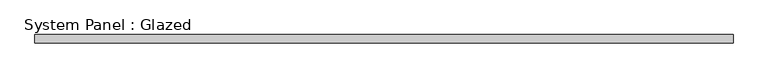
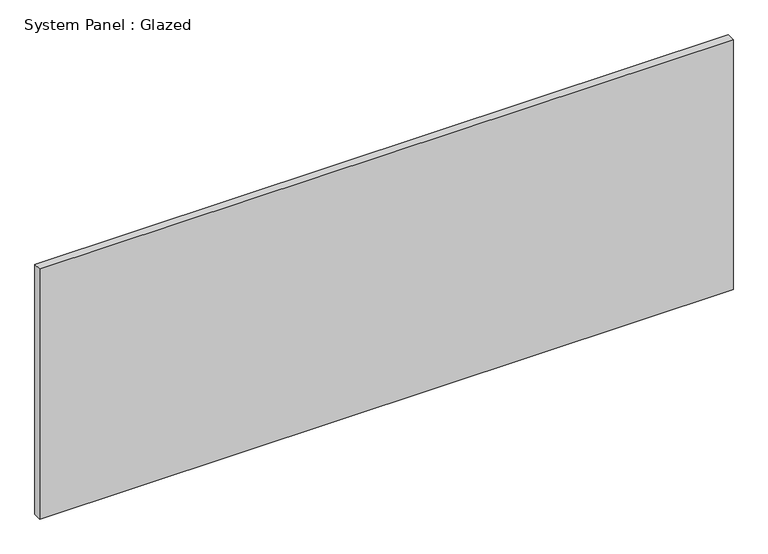
"""IFC4 building model written with IfcOpenShell, lengths in millimetres: plate geometry, System Panel : Glazed."""

import ifcopenshell
import ifcopenshell.guid

model = None  # the IFC model being written
_history = None  # IfcOwnerHistory: only IFC2X3 demands one
_inside = {}  # id of a spatial element -> (the spatial element, [elements in it])
_under = {}  # id of a project, library or spatial element -> (it, [spatial elements below it])
_declared = {}  # id of a project -> (the project, [libraries it declares])
_typed = {}  # id of a type object -> (the type object, [elements of that type])
_made_of = {}  # id of a material, layer set ... -> (it, [elements and type objects made of it])


def new_model(schema):
    """Start an empty IFC model of exactly this schema.

    Asked for "IFC4X3", IfcOpenShell would pick the latest addendum, in which some entities
    have other attributes; the version numbers below select the first issue.
    IFC2X3 requires an IfcOwnerHistory on every rooted entity: one is made here for all.
    """
    global model, _history
    if schema == "IFC4X3":
        model = ifcopenshell.file(schema_version=(4, 3, 0, 0))
    else:
        model = ifcopenshell.file(schema=schema)
    _inside.clear()
    _under.clear()
    _declared.clear()
    _typed.clear()
    _made_of.clear()
    _history = None
    if model.schema == "IFC2X3":
        org = make("IfcOrganization", Name="unknown")
        user = make(
            "IfcPersonAndOrganization",
            ThePerson=make("IfcPerson", FamilyName="unknown"),
            TheOrganization=org,
        )
        app = make(
            "IfcApplication",
            ApplicationDeveloper=org,
            Version="unknown",
            ApplicationFullName="unknown",
            ApplicationIdentifier="unknown",
        )
        _history = make(
            "IfcOwnerHistory",
            OwningUser=user,
            OwningApplication=app,
            ChangeAction="ADDED",
            CreationDate=0,
        )
    return model


def make(cls, **values):
    """One entity of the class cls with the attributes given. An attribute that is None is left unset."""
    return model.create_entity(
        cls, **{name: value for name, value in values.items() if value is not None}
    )


def rooted(cls, **values):
    """An entity with a GlobalId (a new one), such as an element, a storey or a relation."""
    return make(cls, GlobalId=ifcopenshell.guid.new(), OwnerHistory=_history, **values)


def si_unit(unit_type, name, prefix=None):
    """IfcSIUnit, for example si_unit("LENGTHUNIT", "METRE", prefix="MILLI")."""
    return make("IfcSIUnit", UnitType=unit_type, Prefix=prefix, Name=name)


def assignment(units):
    """IfcUnitAssignment: the units of a project."""
    return None if units is None else make("IfcUnitAssignment", Units=units)


def point(xyz):
    """IfcCartesianPoint."""
    return None if xyz is None else make("IfcCartesianPoint", Coordinates=xyz)


def direction(xyz):
    """IfcDirection."""
    return None if xyz is None else make("IfcDirection", DirectionRatios=xyz)


def frame(location, z_axis=None, x_axis=None):
    """IfcAxis2Placement3D, a coordinate frame: its origin and axes. An axis left out is left unset."""
    return make(
        "IfcAxis2Placement3D",
        Location=point(location),
        Axis=direction(z_axis),
        RefDirection=direction(x_axis),
    )


def origin():
    """The frame at (0, 0, 0) with its axes left unset."""
    return frame((0.0, 0.0, 0.0))


def origin_with_axes():
    """The frame at (0, 0, 0) with the z axis (0, 0, 1) and the x axis (1, 0, 0) written out."""
    return frame((0.0, 0.0, 0.0), z_axis=(0.0, 0.0, 1.0), x_axis=(1.0, 0.0, 0.0))


def place(relative_to, where):
    """IfcLocalPlacement: puts the frame where relative to a parent placement (None: the world)."""
    return make(
        "IfcLocalPlacement", PlacementRelTo=relative_to, RelativePlacement=where
    )


def context(
    kind, dimensions, precision=None, world=None, true_north=None, identifier=None
):
    """IfcGeometricRepresentationContext, for example the 3D "Model" context."""
    return make(
        "IfcGeometricRepresentationContext",
        ContextIdentifier=identifier,
        ContextType=kind,
        CoordinateSpaceDimension=dimensions,
        Precision=precision,
        WorldCoordinateSystem=world,
        TrueNorth=true_north,
    )


def project(units=None, contexts=None):
    """IfcProject with its units and contexts."""
    return rooted(
        "IfcProject",
        Name="project",
        RepresentationContexts=contexts,
        UnitsInContext=assignment(units),
    )


def spatial(cls, under=None, at=None, **own):
    """A site, building, storey or space (cls), placed at a placement, below another one or the project."""
    s = rooted(cls, ObjectPlacement=at, **own)
    if under is not None:
        _under.setdefault(under.id(), (under, []))[1].append(s)
    return s


def polyline(points):
    """IfcPolyline through the points."""
    return make("IfcPolyline", Points=[point(p) for p in points])


def outline(outer, holes=None, kind="AREA"):
    """IfcArbitraryClosedProfileDef: a profile drawn as a closed curve; with holes, ...WithVoids."""
    if holes is None:
        return make("IfcArbitraryClosedProfileDef", ProfileType=kind, OuterCurve=outer)
    return make(
        "IfcArbitraryProfileDefWithVoids",
        ProfileType=kind,
        OuterCurve=outer,
        InnerCurves=holes,
    )


def extrude(swept, where, along, depth):
    """IfcExtrudedAreaSolid: the profile swept, set in the frame where, extruded along a direction by depth."""
    return make(
        "IfcExtrudedAreaSolid",
        SweptArea=swept,
        Position=where,
        ExtrudedDirection=direction(along),
        Depth=depth,
    )


def shape(context_of_items, identifier, shape_type, items):
    """IfcShapeRepresentation: the items that make up one representation, for example the "Body"."""
    return make(
        "IfcShapeRepresentation",
        ContextOfItems=context_of_items,
        RepresentationIdentifier=identifier,
        RepresentationType=shape_type,
        Items=items,
    )


def source(mapping_origin, context_of_items, identifier, shape_type, items):
    """IfcRepresentationMap: a shape defined once, which mapped items show again and again."""
    return make(
        "IfcRepresentationMap",
        MappingOrigin=mapping_origin,
        MappedRepresentation=shape(context_of_items, identifier, shape_type, items),
    )


def transform(
    local_origin,
    x_axis=None,
    y_axis=None,
    z_axis=None,
    scale=None,
    scale2=None,
    scale3=None,
    uniform=True,
):
    """IfcCartesianTransformationOperator3D, or its non-uniform kind. x_axis, y_axis, z_axis: its Axis1, 2, 3."""
    if uniform:
        return make(
            "IfcCartesianTransformationOperator3D",
            Axis1=direction(x_axis),
            Axis2=direction(y_axis),
            LocalOrigin=point(local_origin),
            Scale=scale,
            Axis3=direction(z_axis),
        )
    return make(
        "IfcCartesianTransformationOperator3DnonUniform",
        Axis1=direction(x_axis),
        Axis2=direction(y_axis),
        LocalOrigin=point(local_origin),
        Scale=scale,
        Axis3=direction(z_axis),
        Scale2=scale2,
        Scale3=scale3,
    )


def mapped(mapping_source, mapping_target):
    """IfcMappedItem: shows the shape of a source again, moved by a transform."""
    return make(
        "IfcMappedItem", MappingSource=mapping_source, MappingTarget=mapping_target
    )


def made_of(thing, what):
    """Note that an element or type object is made of a material, layer set ...; save() writes the relation."""
    if what is not None:
        _made_of.setdefault(what.id(), (what, []))[1].append(thing)
    return thing


def element(
    cls,
    number,
    at=None,
    inside=None,
    cuts=None,
    type_object=None,
    material=None,
    context=None,
    identifier="Body",
    shape_type=None,
    held_by="IfcProductDefinitionShape",
    body=None,
    shapes=None,
    **own,
):
    """One element of the class cls, such as IfcWall. Its Tag is "e" and its number.

    at: its placement. inside: the storey or other place that contains it. cuts: it is an
    opening in that element (IfcRelVoidsElement). A single representation is given by context,
    identifier, shape_type and body (its items); several are given by shapes. held_by: the class
    of the entity that holds the representations. save() writes the other relations.
    """
    e = rooted(cls, Tag="e%d" % number, ObjectPlacement=at, **own)
    if body is not None:
        shapes = [shape(context, identifier, shape_type, body)]
    if shapes is not None:
        e.Representation = make(held_by, Representations=shapes)
    if inside is not None:
        _inside.setdefault(inside.id(), (inside, []))[1].append(e)
    if cuts is not None:
        rooted(
            "IfcRelVoidsElement", RelatingBuildingElement=cuts, RelatedOpeningElement=e
        )
    if type_object is not None:
        _typed.setdefault(type_object.id(), (type_object, []))[1].append(e)
    return made_of(e, material)


def aggregate(whole, parts):
    """IfcRelAggregates: a whole, such as a stair, and the parts it consists of."""
    return rooted("IfcRelAggregates", RelatingObject=whole, RelatedObjects=parts)


def save(model, path):
    """Write the relations noted so far, then the file.

    IfcRelAggregates (storeys below a building ...), IfcRelContainedInSpatialStructure (elements
    in a storey), IfcRelDefinesByType, IfcRelAssociatesMaterial and IfcRelDeclares: one each for
    every whole, place, type object, material and project.
    """
    for whole, parts in _under.values():
        aggregate(whole, parts)
    for where, things in _inside.values():
        rooted(
            "IfcRelContainedInSpatialStructure",
            RelatedElements=things,
            RelatingStructure=where,
        )
    for kind, things in _typed.values():
        rooted("IfcRelDefinesByType", RelatedObjects=things, RelatingType=kind)
    for what, things in _made_of.values():
        rooted("IfcRelAssociatesMaterial", RelatedObjects=things, RelatingMaterial=what)
    for by, libraries in _declared.values():
        rooted("IfcRelDeclares", RelatingContext=by, RelatedDefinitions=libraries)
    model.write(path)


def system_panel_glazed_ad6e6b44(model_context):
    return source(origin(), model_context, "Body", "SweptSolid", [
        extrude(outline(polyline([(1073.15, -44.45), (-1073.15, -44.45), (-1073.15, -19.05), (1073.15, -19.05), (1073.15, -44.45)])), origin_with_axes(), (0.0, 0.0, 1.0), 819.15),
    ])


if __name__ == "__main__":
    model = new_model("IFC4")
    model_context = context("Model", 3, world=origin())
    ifc_project = project(units=[si_unit("LENGTHUNIT", "METRE", prefix="MILLI")], contexts=[model_context])
    site = spatial("IfcSite", under=ifc_project)
    building = spatial("IfcBuilding", under=site)
    placement = place(None, origin())
    system_panel_glazed_shape = system_panel_glazed_ad6e6b44(model_context)
    element("IfcPlate", 1, ObjectType="System Panel : Glazed", at=placement, inside=building, context=model_context, shape_type="MappedRepresentation", body=[
        mapped(system_panel_glazed_shape, transform((0.0, 0.0, 0.0), x_axis=(1.0, 0.0, 0.0), y_axis=(0.0, 1.0, 0.0), z_axis=(0.0, 0.0, 1.0))),
    ])
    save(model, "model.ifc")

# Revit data of these elements
# Type "System Panel : Glazed"
#   Construction Type Id = "GSP4R"
#   Analytic Construction = "1/8 in Pilkington single glazing"
#   Visual Light Transmittance = 0.9
#   Solar Heat Gain Coefficient = 0.86
#   Heat Transfer Coefficient (U) = 1.18115 BTU/(h·ft²·°F)
#   Define Thermal Properties by = 1
# Element 1 (IfcPlate, "System Panel : Glazed")
#   Materials on its faces: "Glass"
# Materials
#   "Glass": class "Glass", colour RGB 0 128 192, transparency 0.75, Description = "Soda Lime Glass", Cost = 0
